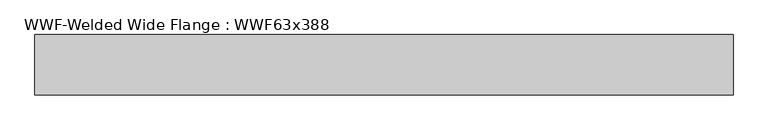
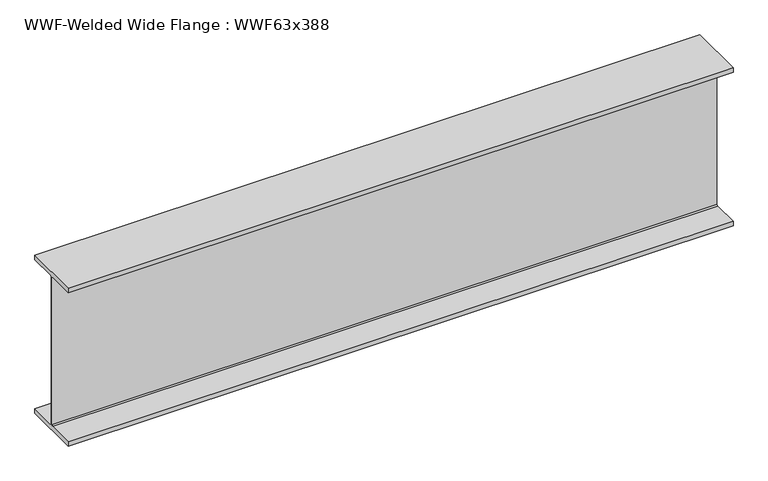
"""IFC4 building model written with IfcOpenShell, lengths in millimetres: beam geometry, WWF-Welded Wide Flange : WWF63x388."""

from ifc_helpers import new_model, si_unit, frame, origin, place, context, project, spatial, polyline, outline, extrude, source, transform, mapped, element, save


def wwf_welded_wide_flange_wwf63x388_85bb2313(model_context):
    return source(origin(), model_context, "Body", "SweptSolid", [
        extrude(outline(polyline([(274.955, -755.015), (274.955, -799.973), (-274.955, -799.973), (-274.955, -755.015), (-19.05, -755.015), (-8.001, -743.966), (-8.001, 743.966), (-19.05, 755.015), (-274.955, 755.015), (-274.955, 799.973), (274.955, 799.973), (274.955, 755.015), (19.05, 755.015), (8.001, 743.966), (8.001, -743.966), (19.05, -755.015), (274.955, -755.015)])), frame((-3184.5707048, 0.0, 0.0), z_axis=(1.0, 0.0, 0.0), x_axis=(0.0, 1.0, 0.0)), (0.0, 0.0, 1.0), 6369.1344444),
    ])


if __name__ == "__main__":
    model = new_model("IFC4")
    model_context = context("Model", 3, world=origin())
    ifc_project = project(units=[si_unit("LENGTHUNIT", "METRE", prefix="MILLI")], contexts=[model_context])
    site = spatial("IfcSite", under=ifc_project)
    building = spatial("IfcBuilding", under=site)
    placement = place(None, origin())
    wwf_welded_wide_flange_wwf63x388_shape = wwf_welded_wide_flange_wwf63x388_85bb2313(model_context)
    element("IfcBeam", 1, ObjectType="WWF-Welded Wide Flange : WWF63x388", at=placement, inside=building, context=model_context, shape_type="MappedRepresentation", body=[
        mapped(wwf_welded_wide_flange_wwf63x388_shape, transform((0.0, 0.0, 0.0), x_axis=(1.0, 0.0, 0.0), y_axis=(0.0, 1.0, 0.0), z_axis=(0.0, 0.0, 1.0))),
    ])
    save(model, "model.ifc")

# Revit data of these elements
# Type "WWF-Welded Wide Flange : WWF63x388"
#   Assembly Code = "B10"
#   Nominal d = "12"
#   W = 388
#   Length [instance default] = 1524 mm
#   bf = 549.91 mm
#   d = 1599.946 mm
#   k = 19.05 mm
#   tf = 44.958 mm
#   tw = 16.002 mm
#   A = 0.0735482 m²
#   Structural Material [instance default] = Steel ASTM A572
# Element 1 (IfcBeam, "WWF-Welded Wide Flange : WWF63x388")
#   Structural Material = Metal - Steel 43-275
#   Materials on its faces: "Metal - Steel 43-275"
# Materials
#   "Steel ASTM A572": class "Metal", colour RGB 247 247 247, transparency 0, Description = "Structural steel, high strength low alloy, ASTM - A572 - 50", Cost = 0
#   "Metal - Steel 43-275": class "Metal", colour RGB 247 247 247, transparency 0, Cost = 0
